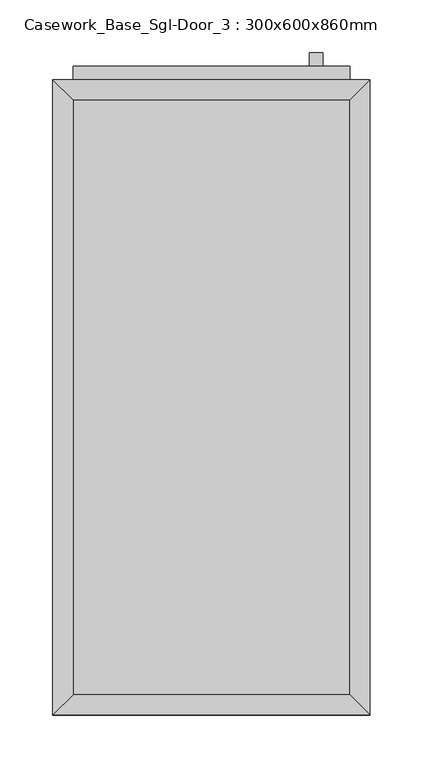
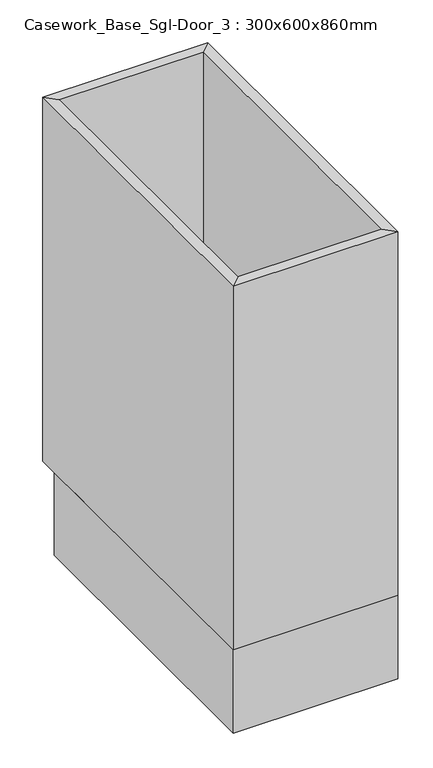
"""IFC4 building model written with IfcOpenShell, lengths in millimetres: furniture geometry, Casework_Base_Sgl-Door_3 : 300x600x860mm."""

from ifc_helpers import new_model, si_unit, frame, origin, origin_with_axes, place, context, project, spatial, polyline, outline, extrude, faceted_brep, source, transform, mapped, element, save


def casework_base_sgl_door_3_300x600x860mm_7fc0b309(model_context):
    return source(origin(), model_context, "Body", "SolidModel", [
        extrude(outline(polyline([(149.6877049, 19.05), (-112.2122951, 19.05), (-112.2122951, 580.95), (149.6877049, 580.95), (149.6877049, 19.05)])), frame((0.0, 0.0, 160.0), z_axis=(0.0, 0.0, 1.0), x_axis=(1.0, 0.0, 0.0)), (0.0, 0.0, 1.0), 19.05),
        faceted_brep([(149.6877049, 580.95, 860.0), (-112.2122951, 580.95, 860.0), (-112.2122951, 580.95, 160.0), (149.6877049, 580.95, 160.0), (168.7377049, 600.0, 860.0), (-131.2622951, 600.0, 860.0), (168.7377049, 600.0, 160.0), (-131.2622951, 600.0, 160.0), (-112.2122951, 19.05, 860.0), (-112.2122951, 19.05, 160.0), (-131.2622951, 0.0, 860.0), (-131.2622951, 0.0, 160.0), (149.6877049, 19.05, 860.0), (149.6877049, 19.05, 160.0), (168.7377049, 0.0, 860.0), (168.7377049, 0.0, 160.0)], [[[0, 1, 2, 3]], [[4, 5, 1, 0]], [[6, 7, 5, 4]], [[3, 2, 7, 6]], [[1, 8, 9, 2]], [[5, 10, 8, 1]], [[7, 11, 10, 5]], [[2, 9, 11, 7]], [[8, 12, 13, 9]], [[10, 14, 12, 8]], [[11, 15, 14, 10]], [[9, 13, 15, 11]], [[12, 0, 3, 13]], [[14, 4, 0, 12]], [[15, 6, 4, 14]], [[13, 3, 6, 15]]]),
        extrude(outline(polyline([(168.7377049, 0.0), (-131.2622951, 0.0), (-131.2622951, 565.0), (168.7377049, 565.0), (168.7377049, 0.0)])), origin_with_axes(), (0.0, 0.0, 1.0), 160.0),
        extrude(outline(polyline([(124.2877049, 625.4), (124.2877049, 612.7), (111.5877049, 612.7), (111.5877049, 625.4), (124.2877049, 625.4)])), frame((0.0, 0.0, 701.25), z_axis=(0.0, 0.0, 1.0), x_axis=(1.0, 0.0, 0.0)), (0.0, 0.0, 1.0), 101.6),
        extrude(outline(polyline([(149.6877049, 612.7), (149.6877049, 600.0), (-112.2122951, 600.0), (-112.2122951, 612.7), (149.6877049, 612.7)])), frame((0.0, 0.0, 179.05), z_axis=(0.0, 0.0, 1.0), x_axis=(1.0, 0.0, 0.0)), (0.0, 0.0, 1.0), 661.9),
    ])


if __name__ == "__main__":
    model = new_model("IFC4")
    model_context = context("Model", 3, world=origin())
    ifc_project = project(units=[si_unit("LENGTHUNIT", "METRE", prefix="MILLI")], contexts=[model_context])
    site = spatial("IfcSite", under=ifc_project)
    building = spatial("IfcBuilding", under=site)
    placement = place(None, origin())
    casework_base_sgl_door_3_300x600x860mm_shape = casework_base_sgl_door_3_300x600x860mm_7fc0b309(model_context)
    element("IfcFurniture", 1, ObjectType="Casework_Base_Sgl-Door_3 : 300x600x860mm", at=placement, inside=building, context=model_context, shape_type="MappedRepresentation", body=[
        mapped(casework_base_sgl_door_3_300x600x860mm_shape, transform((0.0, 0.0, 0.0), x_axis=(1.0, 0.0, 0.0), y_axis=(0.0, 1.0, 0.0), z_axis=(0.0, 0.0, 1.0))),
    ])
    save(model, "model.ifc")

# Revit data of these elements
# Type "Casework_Base_Sgl-Door_3 : 300x600x860mm"
#   Keynote = "N10"
#   Depth = 600 mm
#   Height = 860 mm
#   Plinth Depth = 35 mm
#   Plinth Height = 160 mm
#   Width = 300 mm
#   Material Cabinet = Cabinets
#   Material Door/Drawer = Cabinets
#   Material Handle = Cabinets - Handles
# Element 1 (IfcFurniture, "Casework_Base_Sgl-Door_3 : 300x600x860mm")
#   Materials on its faces: "Cabinets", "Cabinets - Handles"
# Materials
#   "Cabinets": class "Miscellaneous", colour RGB 249 249 249, transparency 0
#   "Cabinets - Handles": class "Metal", colour RGB 57 57 57, transparency 0
